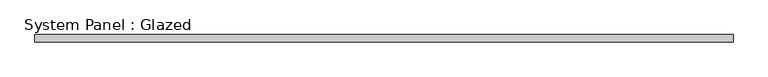
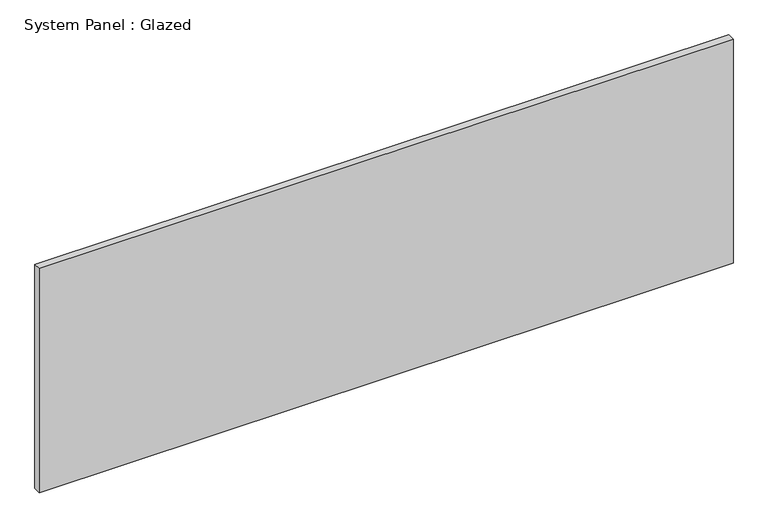
"""IFC4 building model written with IfcOpenShell, lengths in millimetres: plate geometry, System Panel : Glazed."""

import ifcopenshell
import ifcopenshell.guid

model = None  # the IFC model being written
_history = None  # IfcOwnerHistory: only IFC2X3 demands one
_inside = {}  # id of a spatial element -> (the spatial element, [elements in it])
_under = {}  # id of a project, library or spatial element -> (it, [spatial elements below it])
_declared = {}  # id of a project -> (the project, [libraries it declares])
_typed = {}  # id of a type object -> (the type object, [elements of that type])
_made_of = {}  # id of a material, layer set ... -> (it, [elements and type objects made of it])


def new_model(schema):
    """Start an empty IFC model of exactly this schema.

    Asked for "IFC4X3", IfcOpenShell would pick the latest addendum, in which some entities
    have other attributes; the version numbers below select the first issue.
    IFC2X3 requires an IfcOwnerHistory on every rooted entity: one is made here for all.
    """
    global model, _history
    if schema == "IFC4X3":
        model = ifcopenshell.file(schema_version=(4, 3, 0, 0))
    else:
        model = ifcopenshell.file(schema=schema)
    _inside.clear()
    _under.clear()
    _declared.clear()
    _typed.clear()
    _made_of.clear()
    _history = None
    if model.schema == "IFC2X3":
        org = make("IfcOrganization", Name="unknown")
        user = make(
            "IfcPersonAndOrganization",
            ThePerson=make("IfcPerson", FamilyName="unknown"),
            TheOrganization=org,
        )
        app = make(
            "IfcApplication",
            ApplicationDeveloper=org,
            Version="unknown",
            ApplicationFullName="unknown",
            ApplicationIdentifier="unknown",
        )
        _history = make(
            "IfcOwnerHistory",
            OwningUser=user,
            OwningApplication=app,
            ChangeAction="ADDED",
            CreationDate=0,
        )
    return model


def make(cls, **values):
    """One entity of the class cls with the attributes given. An attribute that is None is left unset."""
    return model.create_entity(
        cls, **{name: value for name, value in values.items() if value is not None}
    )


def rooted(cls, **values):
    """An entity with a GlobalId (a new one), such as an element, a storey or a relation."""
    return make(cls, GlobalId=ifcopenshell.guid.new(), OwnerHistory=_history, **values)


def si_unit(unit_type, name, prefix=None):
    """IfcSIUnit, for example si_unit("LENGTHUNIT", "METRE", prefix="MILLI")."""
    return make("IfcSIUnit", UnitType=unit_type, Prefix=prefix, Name=name)


def assignment(units):
    """IfcUnitAssignment: the units of a project."""
    return None if units is None else make("IfcUnitAssignment", Units=units)


def point(xyz):
    """IfcCartesianPoint."""
    return None if xyz is None else make("IfcCartesianPoint", Coordinates=xyz)


def direction(xyz):
    """IfcDirection."""
    return None if xyz is None else make("IfcDirection", DirectionRatios=xyz)


def frame(location, z_axis=None, x_axis=None):
    """IfcAxis2Placement3D, a coordinate frame: its origin and axes. An axis left out is left unset."""
    return make(
        "IfcAxis2Placement3D",
        Location=point(location),
        Axis=direction(z_axis),
        RefDirection=direction(x_axis),
    )


def origin():
    """The frame at (0, 0, 0) with its axes left unset."""
    return frame((0.0, 0.0, 0.0))


def origin_with_axes():
    """The frame at (0, 0, 0) with the z axis (0, 0, 1) and the x axis (1, 0, 0) written out."""
    return frame((0.0, 0.0, 0.0), z_axis=(0.0, 0.0, 1.0), x_axis=(1.0, 0.0, 0.0))


def place(relative_to, where):
    """IfcLocalPlacement: puts the frame where relative to a parent placement (None: the world)."""
    return make(
        "IfcLocalPlacement", PlacementRelTo=relative_to, RelativePlacement=where
    )


def context(
    kind, dimensions, precision=None, world=None, true_north=None, identifier=None
):
    """IfcGeometricRepresentationContext, for example the 3D "Model" context."""
    return make(
        "IfcGeometricRepresentationContext",
        ContextIdentifier=identifier,
        ContextType=kind,
        CoordinateSpaceDimension=dimensions,
        Precision=precision,
        WorldCoordinateSystem=world,
        TrueNorth=true_north,
    )


def project(units=None, contexts=None):
    """IfcProject with its units and contexts."""
    return rooted(
        "IfcProject",
        Name="project",
        RepresentationContexts=contexts,
        UnitsInContext=assignment(units),
    )


def spatial(cls, under=None, at=None, **own):
    """A site, building, storey or space (cls), placed at a placement, below another one or the project."""
    s = rooted(cls, ObjectPlacement=at, **own)
    if under is not None:
        _under.setdefault(under.id(), (under, []))[1].append(s)
    return s


def polyline(points):
    """IfcPolyline through the points."""
    return make("IfcPolyline", Points=[point(p) for p in points])


def outline(outer, holes=None, kind="AREA"):
    """IfcArbitraryClosedProfileDef: a profile drawn as a closed curve; with holes, ...WithVoids."""
    if holes is None:
        return make("IfcArbitraryClosedProfileDef", ProfileType=kind, OuterCurve=outer)
    return make(
        "IfcArbitraryProfileDefWithVoids",
        ProfileType=kind,
        OuterCurve=outer,
        InnerCurves=holes,
    )


def extrude(swept, where, along, depth):
    """IfcExtrudedAreaSolid: the profile swept, set in the frame where, extruded along a direction by depth."""
    return make(
        "IfcExtrudedAreaSolid",
        SweptArea=swept,
        Position=where,
        ExtrudedDirection=direction(along),
        Depth=depth,
    )


def shape(context_of_items, identifier, shape_type, items):
    """IfcShapeRepresentation: the items that make up one representation, for example the "Body"."""
    return make(
        "IfcShapeRepresentation",
        ContextOfItems=context_of_items,
        RepresentationIdentifier=identifier,
        RepresentationType=shape_type,
        Items=items,
    )


def source(mapping_origin, context_of_items, identifier, shape_type, items):
    """IfcRepresentationMap: a shape defined once, which mapped items show again and again."""
    return make(
        "IfcRepresentationMap",
        MappingOrigin=mapping_origin,
        MappedRepresentation=shape(context_of_items, identifier, shape_type, items),
    )


def transform(
    local_origin,
    x_axis=None,
    y_axis=None,
    z_axis=None,
    scale=None,
    scale2=None,
    scale3=None,
    uniform=True,
):
    """IfcCartesianTransformationOperator3D, or its non-uniform kind. x_axis, y_axis, z_axis: its Axis1, 2, 3."""
    if uniform:
        return make(
            "IfcCartesianTransformationOperator3D",
            Axis1=direction(x_axis),
            Axis2=direction(y_axis),
            LocalOrigin=point(local_origin),
            Scale=scale,
            Axis3=direction(z_axis),
        )
    return make(
        "IfcCartesianTransformationOperator3DnonUniform",
        Axis1=direction(x_axis),
        Axis2=direction(y_axis),
        LocalOrigin=point(local_origin),
        Scale=scale,
        Axis3=direction(z_axis),
        Scale2=scale2,
        Scale3=scale3,
    )


def mapped(mapping_source, mapping_target):
    """IfcMappedItem: shows the shape of a source again, moved by a transform."""
    return make(
        "IfcMappedItem", MappingSource=mapping_source, MappingTarget=mapping_target
    )


def made_of(thing, what):
    """Note that an element or type object is made of a material, layer set ...; save() writes the relation."""
    if what is not None:
        _made_of.setdefault(what.id(), (what, []))[1].append(thing)
    return thing


def element(
    cls,
    number,
    at=None,
    inside=None,
    cuts=None,
    type_object=None,
    material=None,
    context=None,
    identifier="Body",
    shape_type=None,
    held_by="IfcProductDefinitionShape",
    body=None,
    shapes=None,
    **own,
):
    """One element of the class cls, such as IfcWall. Its Tag is "e" and its number.

    at: its placement. inside: the storey or other place that contains it. cuts: it is an
    opening in that element (IfcRelVoidsElement). A single representation is given by context,
    identifier, shape_type and body (its items); several are given by shapes. held_by: the class
    of the entity that holds the representations. save() writes the other relations.
    """
    e = rooted(cls, Tag="e%d" % number, ObjectPlacement=at, **own)
    if body is not None:
        shapes = [shape(context, identifier, shape_type, body)]
    if shapes is not None:
        e.Representation = make(held_by, Representations=shapes)
    if inside is not None:
        _inside.setdefault(inside.id(), (inside, []))[1].append(e)
    if cuts is not None:
        rooted(
            "IfcRelVoidsElement", RelatingBuildingElement=cuts, RelatedOpeningElement=e
        )
    if type_object is not None:
        _typed.setdefault(type_object.id(), (type_object, []))[1].append(e)
    return made_of(e, material)


def aggregate(whole, parts):
    """IfcRelAggregates: a whole, such as a stair, and the parts it consists of."""
    return rooted("IfcRelAggregates", RelatingObject=whole, RelatedObjects=parts)


def save(model, path):
    """Write the relations noted so far, then the file.

    IfcRelAggregates (storeys below a building ...), IfcRelContainedInSpatialStructure (elements
    in a storey), IfcRelDefinesByType, IfcRelAssociatesMaterial and IfcRelDeclares: one each for
    every whole, place, type object, material and project.
    """
    for whole, parts in _under.values():
        aggregate(whole, parts)
    for where, things in _inside.values():
        rooted(
            "IfcRelContainedInSpatialStructure",
            RelatedElements=things,
            RelatingStructure=where,
        )
    for kind, things in _typed.values():
        rooted("IfcRelDefinesByType", RelatedObjects=things, RelatingType=kind)
    for what, things in _made_of.values():
        rooted("IfcRelAssociatesMaterial", RelatedObjects=things, RelatingMaterial=what)
    for by, libraries in _declared.values():
        rooted("IfcRelDeclares", RelatingContext=by, RelatedDefinitions=libraries)
    model.write(path)


def system_panel_glazed_4fe69e40(model_context):
    return source(origin(), model_context, "Body", "SweptSolid", [
        extrude(outline(polyline([(1199.1815359, -44.45), (-1199.1815359, -44.45), (-1199.1815359, -19.05), (1199.1815359, -19.05), (1199.1815359, -44.45)])), origin_with_axes(), (0.0, 0.0, 1.0), 819.15),
    ])


if __name__ == "__main__":
    model = new_model("IFC4")
    model_context = context("Model", 3, world=origin())
    ifc_project = project(units=[si_unit("LENGTHUNIT", "METRE", prefix="MILLI")], contexts=[model_context])
    site = spatial("IfcSite", under=ifc_project)
    building = spatial("IfcBuilding", under=site)
    placement = place(None, origin())
    system_panel_glazed_shape = system_panel_glazed_4fe69e40(model_context)
    element("IfcPlate", 1, ObjectType="System Panel : Glazed", at=placement, inside=building, context=model_context, shape_type="MappedRepresentation", body=[
        mapped(system_panel_glazed_shape, transform((0.0, 0.0, 0.0), x_axis=(1.0, 0.0, 0.0), y_axis=(0.0, 1.0, 0.0), z_axis=(0.0, 0.0, 1.0))),
    ])
    save(model, "model.ifc")

# Revit data of these elements
# Type "System Panel : Glazed"
#   Construction Type Id = "GSP4R"
#   Analytic Construction = "1/8 in Pilkington single glazing"
#   Visual Light Transmittance = 0.9
#   Solar Heat Gain Coefficient = 0.86
#   Heat Transfer Coefficient (U) = 1.18115 BTU/(h·ft²·°F)
#   Define Thermal Properties by = 1
# Element 1 (IfcPlate, "System Panel : Glazed")
#   Materials on its faces: "Glass"
# Materials
#   "Glass": class "Glass", colour RGB 0 128 192, transparency 0.75, Description = "Soda Lime Glass", Cost = 0
